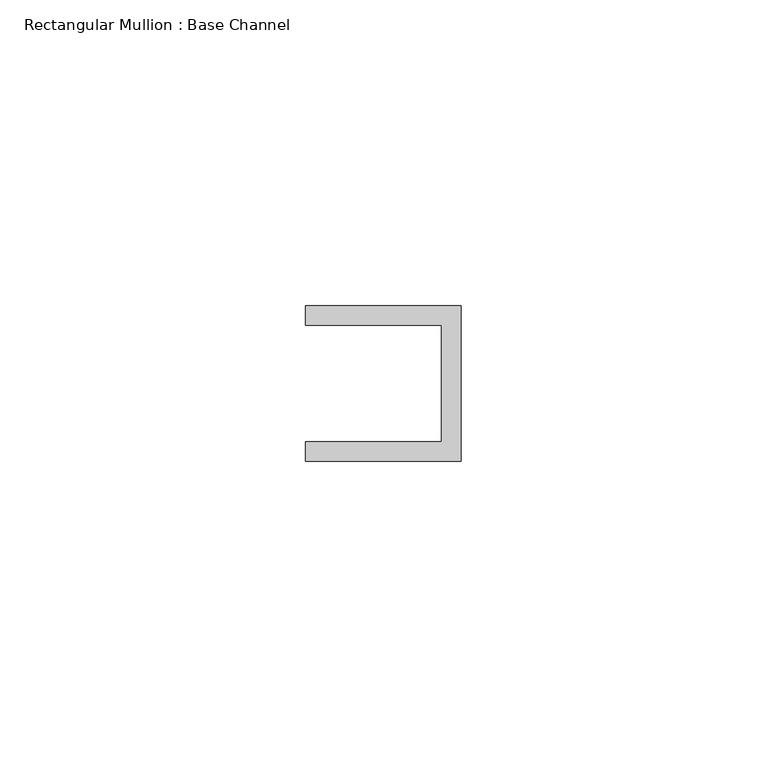
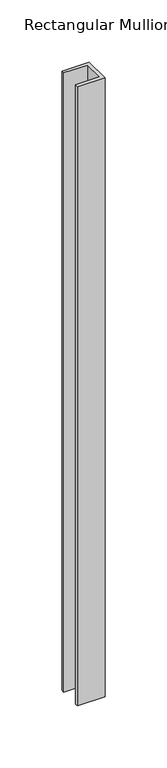
"""IFC4 building model written with IfcOpenShell, lengths in millimetres: member geometry, Rectangular Mullion : Base Channel."""

from ifc_helpers import new_model, si_unit, frame, origin, place, context, project, spatial, polyline, outline, extrude, source, transform, mapped, element, save


def rectangular_mullion_base_channel_60826c86(model_context):
    return source(origin(), model_context, "Body", "SweptSolid", [
        extrude(outline(polyline([(0.0, 12.7), (0.0, -12.7), (-25.4, -12.7), (-25.4, -9.525), (-3.175, -9.525), (-3.175, 9.525), (-25.4, 9.525), (-25.4, 12.7), (0.0, 12.7)])), frame((0.0, 0.0, -609.6), z_axis=(0.0, 0.0, 1.0), x_axis=(1.0, 0.0, 0.0)), (0.0, 0.0, 1.0), 609.6),
    ])


if __name__ == "__main__":
    model = new_model("IFC4")
    model_context = context("Model", 3, world=origin())
    ifc_project = project(units=[si_unit("LENGTHUNIT", "METRE", prefix="MILLI")], contexts=[model_context])
    site = spatial("IfcSite", under=ifc_project)
    building = spatial("IfcBuilding", under=site)
    placement = place(None, origin())
    rectangular_mullion_base_channel_shape = rectangular_mullion_base_channel_60826c86(model_context)
    element("IfcMember", 1, ObjectType="Rectangular Mullion : Base Channel", at=placement, inside=building, context=model_context, shape_type="MappedRepresentation", body=[
        mapped(rectangular_mullion_base_channel_shape, transform((0.0, 0.0, 0.0), x_axis=(1.0, 0.0, 0.0), y_axis=(0.0, 1.0, 0.0), z_axis=(0.0, 0.0, 1.0))),
    ])
    save(model, "model.ifc")

# Revit data of these elements
# Type "Rectangular Mullion : Base Channel"
#   built-in parameter 1007322 = 0.0833333 (stored number, unit not read)
#   built-in parameter 1007321 = 0.0416667 (stored number, unit not read)
#   built-in parameter 1007320 = -0.03125 (stored number, unit not read)
# Element 1 (IfcMember, "Rectangular Mullion : Base Channel")
#   Materials on its faces: "ALUM"
# Materials
#   "ALUM": class "Generic", colour RGB 157 157 157, transparency 0, Cost = 0
